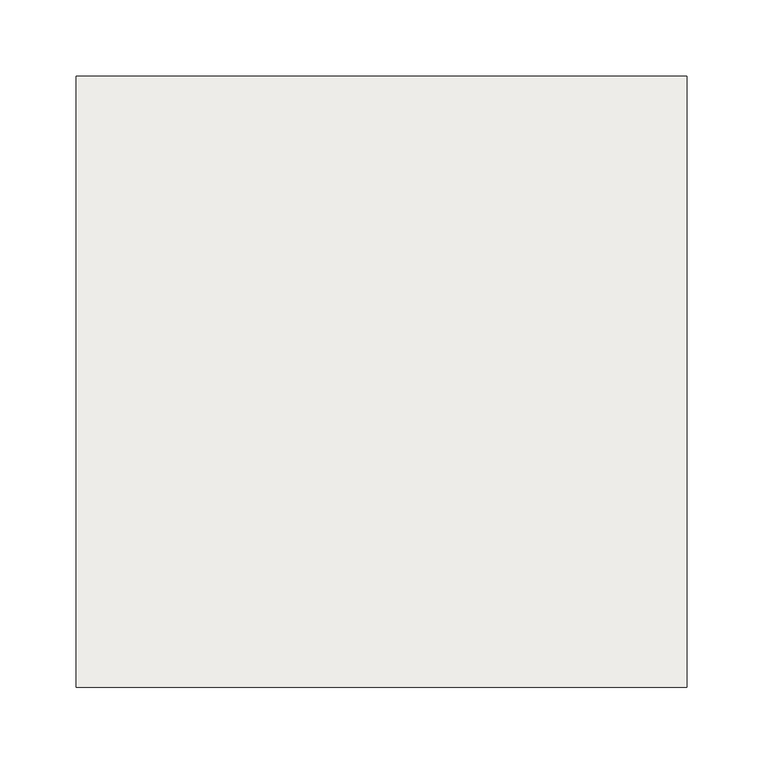
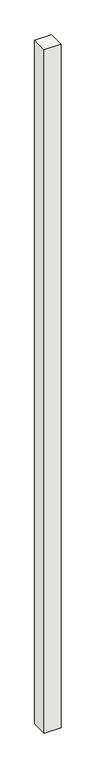
"""IFC4 building model written with IfcOpenShell, lengths in millimetres: footing geometry, NLRS_17_SFO_TLB_funderingspaal geheid beton prefab-AV-MMBPC_gen_rsf : heipaal beton prefab_gen__bxh 400x400."""

from ifc_helpers import new_model, si_unit, frame, origin, place, context, project, spatial, polyline, outline, extrude, source, transform, mapped, element, save


def footing_73a1868d(model_context):
    return source(origin(), model_context, "Body", "SweptSolid", [
        extrude(outline(polyline([(200.0, -200.0), (-200.0, -200.0), (-200.0, 200.0), (200.0, 200.0), (200.0, -200.0)])), frame((0.0, 0.0, -20000.0), z_axis=(0.0, 0.0, 1.0), x_axis=(1.0, 0.0, 0.0)), (0.0, 0.0, 1.0), 17400.0),
    ])


if __name__ == "__main__":
    model = new_model("IFC4")
    model_context = context("Model", 3, world=origin())
    ifc_project = project(units=[si_unit("LENGTHUNIT", "METRE", prefix="MILLI")], contexts=[model_context])
    site = spatial("IfcSite", under=ifc_project)
    building = spatial("IfcBuilding", under=site)
    placement = place(None, origin())
    footing_shape = footing_73a1868d(model_context)
    element("IfcFooting", 1, ObjectType="NLRS_17_SFO_TLB_funderingspaal geheid beton prefab-AV-MMBPC_gen_rsf : heipaal beton prefab_gen__bxh 400x400", at=placement, inside=building, context=model_context, shape_type="MappedRepresentation", body=[
        mapped(footing_shape, transform((0.0, 0.0, 0.0), x_axis=(1.0, 0.0, 0.0), y_axis=(0.0, 1.0, 0.0), z_axis=(0.0, 0.0, 1.0))),
    ])
    save(model, "model.ifc")

# Revit data of these elements
# Type "NLRS_17_SFO_TLB_funderingspaal geheid beton prefab-AV-MMBPC_gen_rsf : heipaal beton prefab_gen__bxh 400x400"
#   IfcExportAs = "IfcPile"
#   Type Comments = "prefab heipaal 400x400"
#   Model = " "
#   Manufacturer = " "
#   Description = "prefab heipaal 400x400"
#   Assembly Code = "17.21"
#   Width = 400 mm
#   Slanted Angle [instance default] = 0.00°
#   NLRS_S_draagvermogen_trek [instance default] = 0.00 kN
#   NLRS_S_draagvermogen_druk [instance default] = 0.00 kN
#   NLRS_C_lengte [instance default] = 1660 mm
#   NLRS_C_hoogte = 400 mm
#   NLRS_C_breedte = 400 mm
#   Height [instance default] = 1660 mm
#   Length [instance default] = 1660 mm
#   Angle [instance default] = 0.00°
#   Slanted [instance default] = 0
#   Structural Material = NLRS_f2_beton prefab_gen_rsf
#   Keynote = ""
# Element 1 (IfcFooting, "NLRS_17_SFO_TLB_funderingspaal geheid beton prefab-AV-MMBPC_gen_rsf : heipaal beton prefab_gen__bxh 400x400")
#   NLRS_C_lengte = 17400 mm
#   Height = 17400 mm
#   Length = 17400 mm
#   Materials on its faces: "NLRS_f2_beton prefab_gen_rsf"
# Materials
#   "NLRS_f2_beton prefab_gen_rsf": class "F - Niet gebakken kunststeen", colour RGB 129 133 118, transparency 0, Keynote = "f2", Manufacturer = "Revit Standards Foundation", URL = "www.revitstandards.org", Description = "beton prefab", Cost = 0
